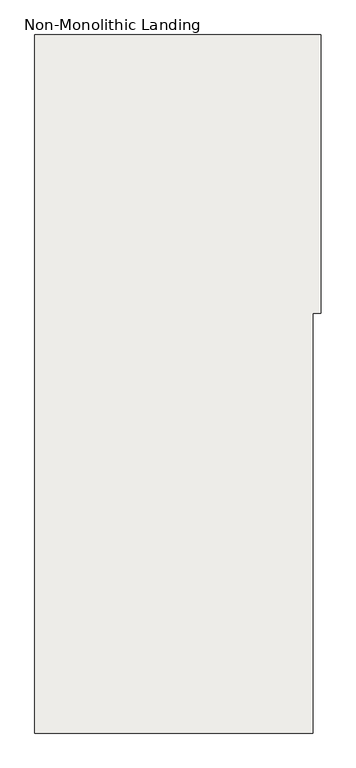
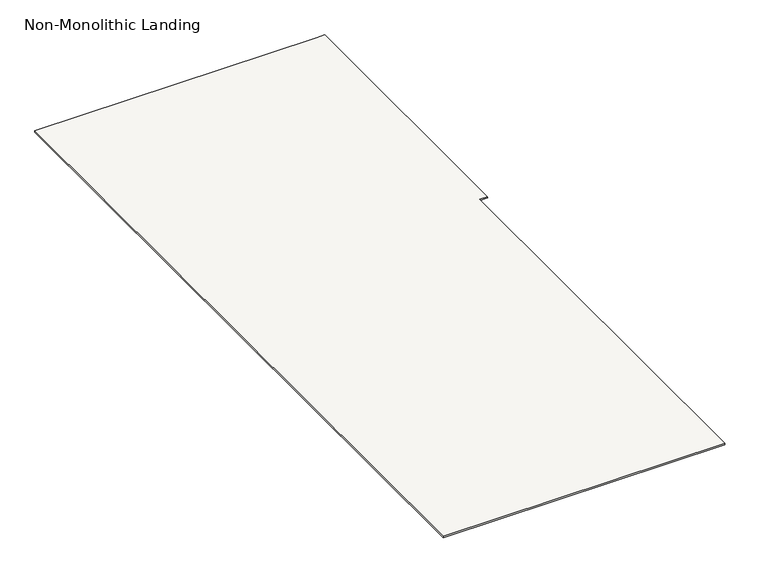
"""IFC4 building model written with IfcOpenShell, lengths in millimetres: slab geometry, Non-Monolithic Landing."""

from ifc_helpers import new_model, si_unit, origin, place, context, project, spatial, faceted_brep, source, transform, mapped, element, save


def non_monolithic_landing_9207be4f(model_context):
    return source(origin(), model_context, "Body", "Brep", [
        faceted_brep([(-16318.9409643, 12030.4345331, 1955.5555556), (-16318.0972143, 12030.4345331, 1949.5555556), (-16318.0972143, 13130.4345331, 1949.5555556), (-16318.9409643, 13130.4345331, 1955.5555556), (-16350.0, 11470.4345331, 1955.5555556), (-16350.0, 12030.4345331, 1955.5555556), (-16350.0, 13130.4345331, 1955.5555556), (-17450.0, 13130.4345331, 1955.5555556), (-17450.0, 10370.4345331, 1955.5555556), (-16350.0, 10370.4345331, 1955.5555556), (-16350.0, 12030.4345331, 1949.5555556), (-16350.0, 11470.4345331, 1949.5555556), (-16350.84375, 11470.4345331, 1949.5555556), (-16350.84375, 10370.4345331, 1949.5555556), (-17450.0, 10370.4345331, 1949.5555556), (-17450.0, 13130.4345331, 1949.5555556), (-16350.0, 13130.4345331, 1949.5555556)], [[[0, 1, 2, 3]], [[4, 5, 0, 3, 6, 7, 8, 9]], [[10, 11, 12, 13, 14, 15, 16, 2, 1]], [[5, 4, 11, 10]], [[0, 5, 10, 1]], [[6, 3, 2, 16]], [[7, 6, 16, 15]], [[8, 7, 15, 14]], [[9, 8, 14, 13]], [[4, 12, 11]], [[12, 4, 9, 13]]]),
    ])


if __name__ == "__main__":
    model = new_model("IFC4")
    model_context = context("Model", 3, world=origin())
    ifc_project = project(units=[si_unit("LENGTHUNIT", "METRE", prefix="MILLI")], contexts=[model_context])
    site = spatial("IfcSite", under=ifc_project)
    building = spatial("IfcBuilding", under=site)
    placement = place(None, origin())
    non_monolithic_landing_shape = non_monolithic_landing_9207be4f(model_context)
    element("IfcSlab", 1, ObjectType="Non-Monolithic Landing", at=placement, inside=building, context=model_context, shape_type="MappedRepresentation", body=[
        mapped(non_monolithic_landing_shape, transform((0.0, 0.0, 0.0), x_axis=(1.0, 0.0, 0.0), y_axis=(0.0, 1.0, 0.0), z_axis=(0.0, 0.0, 1.0))),
    ])
    save(model, "model.ifc")

# Revit data of these elements
# Element 1 (IfcSlab, "Non-Monolithic Landing")
#   Materials on its faces: "Steel, Paint Finish, Dark Gray"
# Materials
#   "Steel, Paint Finish, Dark Gray": class "Metal", colour RGB 89 89 89, transparency 0, Description = "Steel, paint finish, dark gray, glossy", Cost = 0
